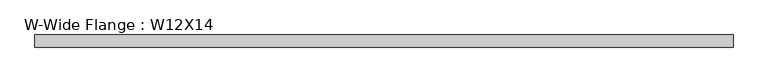
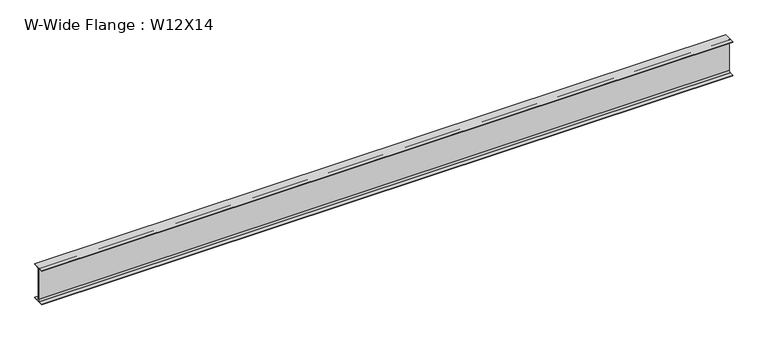
"""IFC4 building model written with IfcOpenShell, lengths in millimetres: beam geometry, W-Wide Flange : W12X14."""

from ifc_helpers import new_model, si_unit, point, frame, frame_2d, origin, place, context, project, spatial, polyline, circle_curve, trimmed, segment, composite_curve, outline, extrude, source, transform, mapped, element, save


def w_wide_flange_w12x14_825a119d(model_context):
    return source(origin(), model_context, "Body", "SweptSolid", [
        extrude(outline(composite_curve([segment(polyline([(50.419, -145.415), (50.419, -151.13), (-50.419, -151.13), (-50.419, -145.415), (-15.875, -145.415)]), True, "CONTINUOUS"), segment(trimmed(circle_curve(frame_2d((-15.875, -132.08)), 13.335), [point((-15.875, -145.415))], [point((-2.54, -132.08))], True, "CARTESIAN"), True, "CONTINUOUS"), segment(polyline([(-2.54, -132.08), (-2.54, 132.08)]), True, "CONTINUOUS"), segment(trimmed(circle_curve(frame_2d((-15.875, 132.08)), 13.335), [point((-2.54, 132.08))], [point((-15.875, 145.415))], True, "CARTESIAN"), True, "CONTINUOUS"), segment(polyline([(-15.875, 145.415), (-50.419, 145.415), (-50.419, 151.13), (50.419, 151.13), (50.419, 145.415), (15.875, 145.415)]), True, "CONTINUOUS"), segment(trimmed(circle_curve(frame_2d((15.875, 132.08)), 13.335), [point((15.875, 145.415))], [point((2.54, 132.08))], True, "CARTESIAN"), True, "CONTINUOUS"), segment(polyline([(2.54, 132.08), (2.54, -132.08)]), True, "CONTINUOUS"), segment(trimmed(circle_curve(frame_2d((15.875, -132.08)), 13.335), [point((2.54, -132.08))], [point((15.875, -145.415))], True, "CARTESIAN"), True, "CONTINUOUS"), segment(polyline([(15.875, -145.415), (50.419, -145.415)]), True, "CONTINUOUS")], self_intersect=False)), frame((-2908.3, 0.0, 0.0), z_axis=(1.0, 0.0, 0.0), x_axis=(0.0, 1.0, 0.0)), (0.0, 0.0, 1.0), 5816.6),
    ])


if __name__ == "__main__":
    model = new_model("IFC4")
    model_context = context("Model", 3, world=origin())
    ifc_project = project(units=[si_unit("LENGTHUNIT", "METRE", prefix="MILLI")], contexts=[model_context])
    site = spatial("IfcSite", under=ifc_project)
    building = spatial("IfcBuilding", under=site)
    placement = place(None, origin())
    w_wide_flange_w12x14_shape = w_wide_flange_w12x14_825a119d(model_context)
    element("IfcBeam", 1, ObjectType="W-Wide Flange : W12X14", at=placement, inside=building, context=model_context, shape_type="MappedRepresentation", body=[
        mapped(w_wide_flange_w12x14_shape, transform((0.0, 0.0, 0.0), x_axis=(1.0, 0.0, 0.0), y_axis=(0.0, 1.0, 0.0), z_axis=(0.0, 0.0, 1.0))),
    ])
    save(model, "model.ifc")

# Revit data of these elements
# Type "W-Wide Flange : W12X14"
#   Assembly Code = "B10"
#   W = 14
#   Length [instance default] = 5' - 0"
#   bf = 0' - 3.97"
#   d = 0' - 11.9"
#   k = 0' - 0 3/4"
#   k2 = 0' - 0.525"
#   tf = 0' - 0.225"
#   tw = 0' - 0.2"
#   A = 0.0288889 SF
#   Structural Material [instance default] = Steel ASTM A992
# Element 1 (IfcBeam, "W-Wide Flange : W12X14")
#   Materials on its faces: "Steel ASTM A992"
# Materials
#   "Steel ASTM A992": class "Metal", colour RGB 199 199 199, transparency 0, Description = "Structural steel 50ksi", Cost = 0
